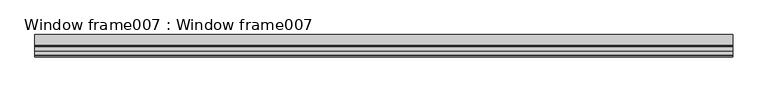
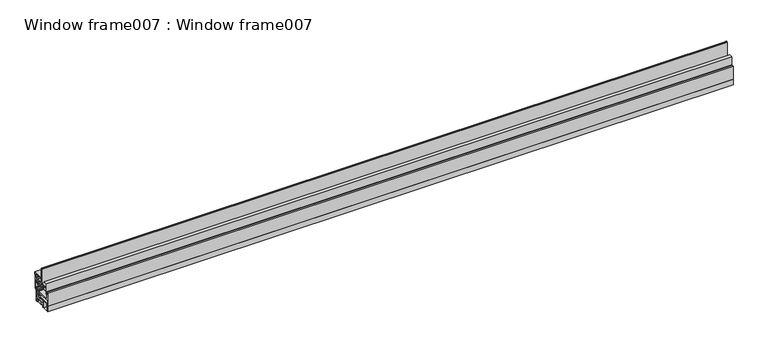
"""IFC4 building model written with IfcOpenShell, lengths in millimetres: proxy geometry, Window frame007 : Window frame007."""

from ifc_helpers import new_model, si_unit, frame, origin, place, context, project, spatial, polyline, outline, extrude, source, transform, mapped, element, save


def window_frame007_window_frame007_a0f1e213(model_context):
    return source(origin(), model_context, "Body", "SweptSolid", [
        extrude(outline(polyline([(-4390.795162, 42521.8453557), (-4390.2197498, 42519.4036919), (-4387.992842, 42519.4036919), (-4387.992842, 42516.9906919), (-4390.219056, 42516.9906919), (-4390.6427973, 42514.531799), (-4391.9961622, 42514.531799), (-4392.6318014, 42517.3937752), (-4392.6318014, 42519.2551381), (-4391.9692743, 42521.8453557), (-4390.795162, 42521.8453557)])), frame((12383.0178845, 0.0, 0.0), z_axis=(1.0, 0.0, 0.0), x_axis=(0.0, 1.0, 0.0)), (0.0, 0.0, 1.0), 2000.0),
        extrude(outline(polyline([(-4420.4203219, 42515.0677418), (-4420.9957341, 42517.5094056), (-4423.222642, 42517.5094056), (-4423.222642, 42519.9224056), (-4420.9964279, 42519.9224056), (-4420.5726866, 42522.3812985), (-4419.2193217, 42522.3812985), (-4418.5836825, 42519.5193223), (-4418.5836825, 42517.6579594), (-4419.2462096, 42515.0677418), (-4420.4203219, 42515.0677418)])), frame((12383.0178845, 0.0, 0.0), z_axis=(1.0, 0.0, 0.0), x_axis=(0.0, 1.0, 0.0)), (0.0, 0.0, 1.0), 2000.0),
        extrude(outline(polyline([(-4437.306942, 42572.6063057), (-4437.306942, 42565.0889235), (-4438.1385224, 42565.0889235), (-4438.1385224, 42568.4642592), (-4441.434442, 42568.4642592), (-4441.434442, 42569.6580592), (-4438.1385224, 42569.6580592), (-4438.1385224, 42572.6063057), (-4437.306942, 42572.6063057)])), frame((12383.0178845, 0.0, 0.0), z_axis=(1.0, 0.0, 0.0), x_axis=(0.0, 1.0, 0.0)), (0.0, 0.0, 1.0), 2000.0),
        extrude(outline(polyline([(-4386.138642, 42549.0568749), (-4386.138642, 42556.574257), (-4385.3070615, 42556.574257), (-4385.3070615, 42553.1989214), (-4382.011142, 42553.1989214), (-4382.011142, 42552.0051214), (-4385.3070615, 42552.0051214), (-4385.3070615, 42549.0568749), (-4386.138642, 42549.0568749)])), frame((12383.0178845, 0.0, 0.0), z_axis=(1.0, 0.0, 0.0), x_axis=(0.0, 1.0, 0.0)), (0.0, 0.0, 1.0), 2000.0),
        extrude(outline(polyline([(-4390.647142, 42598.0807214), (-4380.156942, 42598.0807214), (-4380.156942, 42549.0079214), (-4384.551142, 42549.0079214), (-4384.551142, 42551.2691163), (-4383.281142, 42551.2691163), (-4383.281142, 42550.2779214), (-4382.011142, 42550.2779214), (-4382.011142, 42555.3579214), (-4383.2901234, 42555.3579214), (-4383.2901234, 42554.4695099), (-4384.551142, 42554.4695099), (-4384.551142, 42571.2837214), (-4387.6255994, 42571.2837214), (-4387.6255994, 42573.3157214), (-4385.998942, 42573.3157214), (-4385.998942, 42575.120664), (-4384.5765423, 42575.120664), (-4384.5765423, 42573.3157214), (-4382.188942, 42573.3157214), (-4382.188942, 42582.8214119), (-4384.575932, 42582.8214119), (-4384.575932, 42580.8014104), (-4385.998942, 42580.8014104), (-4385.998942, 42584.8981214), (-4382.188942, 42584.8981214), (-4382.188942, 42596.0487214), (-4390.647142, 42596.0487214), (-4390.647142, 42598.0807214)])), frame((12383.0178845, 0.0, 0.0), z_axis=(1.0, 0.0, 0.0), x_axis=(0.0, 1.0, 0.0)), (0.0, 0.0, 1.0), 2000.0),
        extrude(outline(polyline([(-4400.680142, 42535.1141214), (-4400.680142, 42536.9175214), (-4441.256642, 42536.9175214), (-4441.256642, 42534.8863677), (-4439.8391177, 42532.0915214), (-4443.288642, 42532.0915214), (-4443.288642, 42572.8077214), (-4438.894442, 42572.8077214), (-4438.894442, 42570.5379685), (-4440.1883816, 42570.5379685), (-4440.1883816, 42571.5349778), (-4441.434442, 42571.5349778), (-4441.434442, 42566.4711655), (-4440.1876087, 42566.4711655), (-4440.1876087, 42567.3780411), (-4438.894442, 42567.3780411), (-4438.894442, 42550.5319214), (-4398.330642, 42550.5319214), (-4398.330642, 42547.2547043), (-4399.5842328, 42547.2547043), (-4399.5842328, 42548.4999214), (-4402.140642, 42548.4999214), (-4402.140642, 42538.9495178), (-4397.5514295, 42538.9495178), (-4397.5514295, 42536.9175214), (-4399.2792592, 42536.9175214), (-4399.2792592, 42533.7425214), (-4402.851842, 42533.7425214), (-4402.851842, 42535.1141214), (-4400.680142, 42535.1141214)]), holes=[polyline([(-4440.748642, 42547.3569214), (-4440.748642, 42540.0925214), (-4404.172642, 42540.0925214), (-4404.172642, 42547.3569214), (-4440.748642, 42547.3569214)])]), frame((12383.0178845, 0.0, 0.0), z_axis=(1.0, 0.0, 0.0), x_axis=(0.0, 1.0, 0.0)), (0.0, 0.0, 1.0), 2000.0),
        extrude(outline(polyline([(-4393.9916875, 42527.3417214), (-4418.307742, 42527.3417214), (-4418.307742, 42535.0887214), (-4404.2642819, 42535.0688303), (-4404.2642819, 42533.2201392), (-4397.3509031, 42533.2201392), (-4397.3509031, 42536.9175214), (-4390.532842, 42536.9175214), (-4390.532842, 42533.6388847), (-4392.2263875, 42533.6388847), (-4392.2263875, 42528.8676129), (-4393.9916875, 42527.3417214)])), frame((12383.0178845, 0.0, 0.0), z_axis=(1.0, 0.0, 0.0), x_axis=(0.0, 1.0, 0.0)), (0.0, 0.0, 1.0), 2000.0),
        extrude(outline(polyline([(14383.0178845, -4399.206942), (14383.0178845, -4411.983142), (12383.0178845, -4411.983142), (12383.0178845, -4399.206942), (14383.0178845, -4399.206942)])), frame((0.0, 0.0, 42517.8167214), z_axis=(0.0, 0.0, 1.0), x_axis=(1.0, 0.0, 0.0)), (0.0, 0.0, 1.0), 9.525),
        extrude(outline(polyline([(-4388.170642, 42550.5319214), (-4388.170642, 42555.3579214), (-4386.138642, 42555.3579214), (-4386.138642, 42514.6417214), (-4390.532842, 42514.6417214), (-4390.532842, 42516.895665), (-4389.2906842, 42516.895665), (-4389.2906842, 42515.9117214), (-4387.992842, 42515.9117214), (-4387.992842, 42520.9917214), (-4389.2730298, 42520.9917214), (-4389.2730298, 42520.1283463), (-4390.532842, 42520.1283463), (-4390.532842, 42536.9175214), (-4392.7680416, 42536.9175214), (-4392.7680416, 42538.9495178), (-4388.170642, 42538.9495178), (-4388.170642, 42548.4999214), (-4390.7380948, 42548.4999214), (-4390.7380948, 42547.2410935), (-4391.9593663, 42547.2410935), (-4391.9593663, 42550.5319214), (-4388.170642, 42550.5319214)])), frame((12383.0178845, 0.0, 0.0), z_axis=(1.0, 0.0, 0.0), x_axis=(0.0, 1.0, 0.0)), (0.0, 0.0, 1.0), 2000.0),
        extrude(outline(polyline([(-4393.6152867, 42582.8661214), (-4396.158942, 42582.8661214), (-4396.158942, 42573.3157214), (-4391.5697298, 42573.3157214), (-4391.5697298, 42571.2837214), (-4393.3216328, 42571.2837214), (-4393.3216328, 42568.1087214), (-4397.5578166, 42568.1087214), (-4397.5578166, 42569.4803214), (-4394.6202839, 42569.4803214), (-4394.6202839, 42571.2837214), (-4435.274942, 42571.2837214), (-4435.274942, 42569.0234791), (-4433.8982253, 42566.4577214), (-4437.306942, 42566.4577214), (-4437.306942, 42598.0807214), (-4426.816742, 42598.0807214), (-4426.816742, 42596.0487214), (-4435.274942, 42596.0487214), (-4435.274942, 42584.8981214), (-4413.481742, 42584.8981214), (-4413.481742, 42628.4282541), (-4411.906942, 42628.4282541), (-4411.906942, 42598.1006541), (-4411.9069428, 42584.8981217), (-4392.348942, 42584.8981214), (-4392.348942, 42580.8014104), (-4393.6152867, 42580.8014104), (-4393.6152867, 42582.8661214)]), holes=[polyline([(-4405.1484589, 42574.4587214), (-4398.190942, 42574.4587214), (-4398.190942, 42581.7231214), (-4401.8278546, 42581.7231214), (-4401.8278546, 42582.8661214), (-4411.5992322, 42582.8661214), (-4411.5992322, 42581.7231214), (-4417.3016762, 42581.7231214), (-4417.3016762, 42582.8661214), (-4426.8651528, 42582.8661214), (-4426.8651528, 42581.7231214), (-4430.7855849, 42581.7231214), (-4430.7855849, 42582.8661214), (-4434.766942, 42582.8661214), (-4434.766942, 42573.3157214), (-4430.7398443, 42573.3157214), (-4430.7398443, 42574.4587214), (-4421.8594746, 42574.4587214), (-4421.8594746, 42573.3157214), (-4417.3747372, 42573.3157214), (-4417.3747372, 42574.4587214), (-4413.4782777, 42574.4587214), (-4413.4782777, 42573.3157214), (-4405.1484589, 42573.3157214), (-4405.1484589, 42574.4587214)])]), frame((12383.0178845, 0.0, 0.0), z_axis=(1.0, 0.0, 0.0), x_axis=(0.0, 1.0, 0.0)), (0.0, 0.0, 1.0), 2000.0),
        extrude(outline(polyline([(-4443.288642, 42514.6417214), (-4443.288642, 42532.0915214), (-4439.773833, 42532.0915214), (-4440.7670679, 42534.3350647), (-4439.2720561, 42535.781308), (-4438.4659285, 42535.781308), (-4438.4659285, 42530.6945214), (-4441.891642, 42530.6945214), (-4441.891642, 42516.0387214), (-4424.619642, 42516.0387214), (-4424.619642, 42536.4857214), (-4400.680142, 42536.4857214), (-4400.680142, 42535.1141214), (-4423.222642, 42535.0887214), (-4423.222642, 42522.2778443), (-4420.7028565, 42522.2778443), (-4420.7028565, 42520.0942276), (-4421.876472, 42520.0942276), (-4421.876472, 42520.9917214), (-4423.222642, 42520.9917214), (-4423.222642, 42515.9213761), (-4421.9090714, 42515.9213761), (-4421.9090714, 42516.8504837), (-4420.6702542, 42516.8504837), (-4420.6702542, 42514.6417214), (-4443.288642, 42514.6417214)])), frame((12383.0178845, 0.0, 0.0), z_axis=(1.0, 0.0, 0.0), x_axis=(0.0, 1.0, 0.0)), (0.0, 0.0, 1.0), 2000.0),
        extrude(outline(polyline([(-4411.906942, 42629.8307214), (-4410.890942, 42629.8307214), (-4410.890942, 42599.0967214), (-4379.140942, 42599.0967214), (-4379.140942, 42591.7307214), (-4380.156942, 42591.7307214), (-4380.156942, 42598.0807214), (-4411.906942, 42598.0807214), (-4411.906942, 42629.8307214)])), frame((12383.0178845, 0.0, 0.0), z_axis=(1.0, 0.0, 0.0), x_axis=(0.0, 1.0, 0.0)), (0.0, 0.0, 1.0), 2000.0),
    ])


if __name__ == "__main__":
    model = new_model("IFC4")
    model_context = context("Model", 3, world=origin())
    ifc_project = project(units=[si_unit("LENGTHUNIT", "METRE", prefix="MILLI")], contexts=[model_context])
    site = spatial("IfcSite", under=ifc_project)
    building = spatial("IfcBuilding", under=site)
    placement = place(None, origin())
    window_frame007_window_frame007_shape = window_frame007_window_frame007_a0f1e213(model_context)
    element("IfcBuildingElementProxy", 1, Name="Window frame007 : Window frame007", ObjectType="Window frame007 : Window frame007", at=placement, inside=building, context=model_context, shape_type="MappedRepresentation", body=[
        mapped(window_frame007_window_frame007_shape, transform((0.0, 0.0, 0.0), x_axis=(1.0, 0.0, 0.0), y_axis=(0.0, 1.0, 0.0), z_axis=(0.0, 0.0, 1.0))),
    ])
    save(model, "model.ifc")

# Revit data of these elements
# Type "Window frame007 : Window frame007"
#   NameOverride = "Window frame007"
# Element 1 (IfcBuildingElementProxy, "Window frame007 : Window frame007")
#   Materials on its faces: "FLEETWOOD SERIES 250-T-01 CASEMENT WINDOW FRAME"
# Materials
#   "FLEETWOOD SERIES 250-T-01 CASEMENT WINDOW FRAME": class "Unassigned", colour RGB 128 128 128, transparency 0
